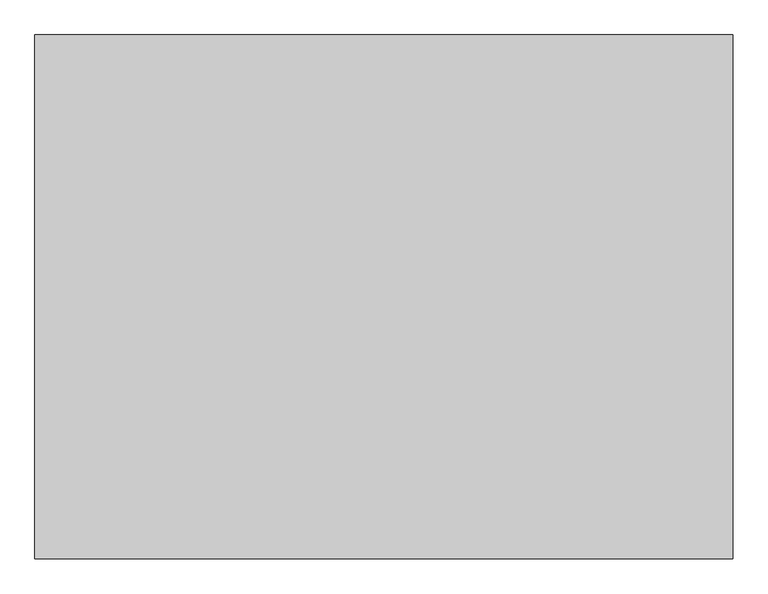
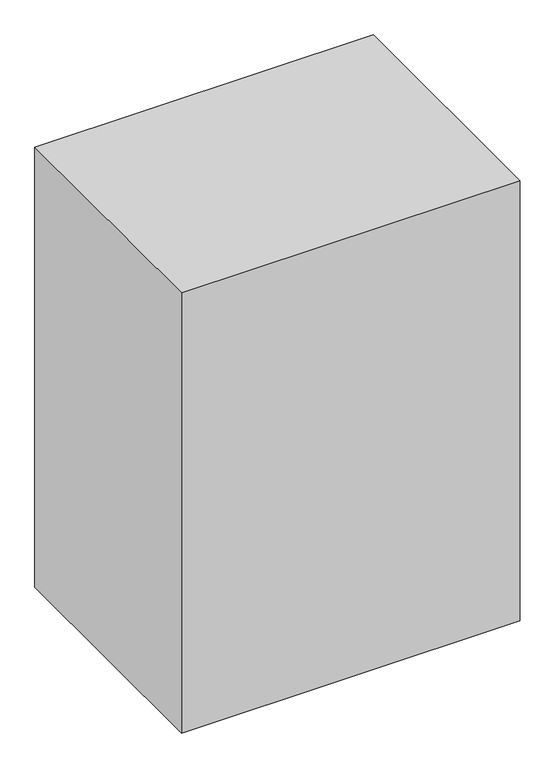
"""IFC4 building model written with IfcOpenShell, lengths in millimetres: proxy geometry, Space Planning Box_hec : Space Planning Box_hec."""

from ifc_helpers import new_model, si_unit, origin, origin_with_axes, place, context, project, spatial, polyline, outline, extrude, source, transform, mapped, element, save


def generic_models_626d8198(model_context):
    return source(origin(), model_context, "Body", "SweptSolid", [
        extrude(outline(polyline([(2000.0, 1500.0), (2000.0, -1500.0), (-2000.0, -1500.0), (-2000.0, 1500.0), (2000.0, 1500.0)])), origin_with_axes(), (0.0, 0.0, 1.0), 5500.0),
    ])


if __name__ == "__main__":
    model = new_model("IFC4")
    model_context = context("Model", 3, world=origin())
    ifc_project = project(units=[si_unit("LENGTHUNIT", "METRE", prefix="MILLI")], contexts=[model_context])
    site = spatial("IfcSite", under=ifc_project)
    building = spatial("IfcBuilding", under=site)
    placement = place(None, origin())
    generic_models_shape = generic_models_626d8198(model_context)
    element("IfcBuildingElementProxy", 1, Name="Space Planning Box_hec : Space Planning Box_hec", ObjectType="Space Planning Box_hec : Space Planning Box_hec", at=placement, inside=building, context=model_context, shape_type="MappedRepresentation", body=[
        mapped(generic_models_shape, transform((0.0, 0.0, 0.0), x_axis=(1.0, 0.0, 0.0), y_axis=(0.0, 1.0, 0.0), z_axis=(0.0, 0.0, 1.0))),
    ])
    save(model, "model.ifc")

# Revit data of these elements
# Type "Space Planning Box_hec : Space Planning Box_hec"
#   Type Comments = "..."
#   Room Name [instance default] = "?"
#   Interior Finish [instance default] = ""
#   Exterior Finish [instance default] = ""
#   Department [instance default] = ""
#   Assembly Code = "..."
#   ceiling height [instance default] = 0
#   Width [instance default] = 1524 mm
#   Program Area [instance default] = 0.00 m²
#   Length [instance default] = 1524 mm
#   Height [instance default] = 1524 mm
#   Area [instance default] = 2.32258 m²
#   Fill Color [instance default] = Cyan
#   Default Elevation = 0
# Element 1 (IfcBuildingElementProxy, "Space Planning Box_hec : Space Planning Box_hec")
#   Room Name = "Elevator"
#   Exterior Finish = "N/A..N/A,,EW2..N/A..N/A"
#   Department = "PATHV2"
#   Width = 4000 mm
#   Program Area = 12.00 m²
#   Length = 3000 mm
#   Height = 5500 mm
#   Area = 12.00 m²
#   Fill Color = Blue
#   Materials on its faces: "Blue"
# Materials
#   "Cyan": class "Generic", colour RGB 0 255 255, transparency 0.2, Cost = 0
#   "Blue": class "Generic", colour RGB 0 0 255, transparency 0.2, Cost = 0
